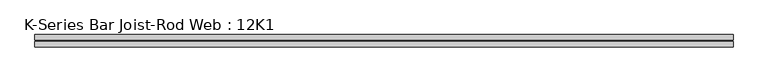
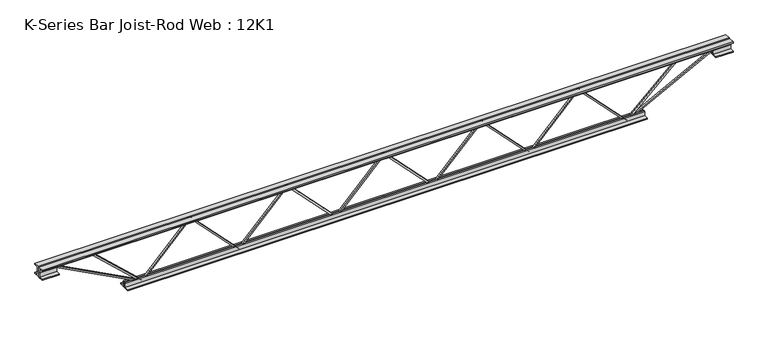
"""IFC4 building model written with IfcOpenShell, lengths in millimetres: beam geometry, K-Series Bar Joist-Rod Web : 12K1."""

from ifc_helpers import new_model, si_unit, frame, origin, place, context, project, spatial, polyline, outline, extrude, source, transform, mapped, element, save


def k_series_bar_joist_rod_web_12k1_6bf771c6(model_context):
    return source(origin(), model_context, "Body", "SweptSolid", [
        extrude(outline(polyline([(-141.2875, 287.02), (-150.8125, 287.02), (-150.8125, 292.22359), (141.2875, 572.89359), (141.2875, 575.18641), (-150.8125, 855.85641), (-150.8125, 861.06), (-141.2875, 861.06), (-141.2875, 859.91359), (150.8125, 579.24359), (150.8125, 568.83641), (-141.2875, 288.16641), (-141.2875, 287.02)])), frame((0.0, -4.7625, 0.0), z_axis=(0.0, 1.0, 0.0), x_axis=(0.0, 0.0, 1.0)), (0.0, 0.0, 1.0), 9.525),
        extrude(outline(polyline([(-141.2875, -287.02), (-150.8125, -287.02), (-150.8125, -281.81641), (141.2875, -1.14641), (141.2875, 1.14641), (-150.8125, 281.81641), (-150.8125, 287.02), (-141.2875, 287.02), (-141.2875, 285.87359), (150.8125, 5.20359), (150.8125, -5.20359), (-141.2875, -285.87359), (-141.2875, -287.02)])), frame((0.0, -4.7625, 0.0), z_axis=(0.0, 1.0, 0.0), x_axis=(0.0, 0.0, 1.0)), (0.0, 0.0, 1.0), 9.525),
        extrude(outline(polyline([(-141.2875, -861.06), (-150.8125, -861.06), (-150.8125, -855.85641), (141.2875, -575.18641), (141.2875, -572.89359), (-150.8125, -292.22359), (-150.8125, -287.02), (-141.2875, -287.02), (-141.2875, -288.16641), (150.8125, -568.83641), (150.8125, -579.24359), (-141.2875, -859.91359), (-141.2875, -861.06)])), frame((0.0, -4.7625, 0.0), z_axis=(0.0, 1.0, 0.0), x_axis=(0.0, 0.0, 1.0)), (0.0, 0.0, 1.0), 9.525),
        extrude(outline(polyline([(-141.2875, 861.06), (-150.8125, 861.06), (-150.8125, 866.26359), (141.2875, 1146.93359), (141.2875, 1149.22641), (-150.8125, 1429.89641), (-150.8125, 1435.1), (-141.2875, 1435.1), (-141.2875, 1433.95359), (150.8125, 1153.28359), (150.8125, 1142.87641), (-141.2875, 862.20641), (-141.2875, 861.06)])), frame((0.0, -4.7625, 0.0), z_axis=(0.0, 1.0, 0.0), x_axis=(0.0, 0.0, 1.0)), (0.0, 0.0, 1.0), 9.525),
        extrude(outline(polyline([(-141.2875, -1435.1), (-150.8125, -1435.1), (-150.8125, -1429.89641), (141.2875, -1149.22641), (141.2875, -1146.93359), (-150.8125, -866.26359), (-150.8125, -861.06), (-141.2875, -861.06), (-141.2875, -862.20641), (150.8125, -1142.87641), (150.8125, -1153.28359), (-141.2875, -1433.95359), (-141.2875, -1435.1)])), frame((0.0, -4.7625, 0.0), z_axis=(0.0, 1.0, 0.0), x_axis=(0.0, 0.0, 1.0)), (0.0, 0.0, 1.0), 9.525),
        extrude(outline(polyline([(4.7625, 152.4), (36.5125, 152.4), (36.5125, 146.05), (11.1125, 146.05), (11.1125, 120.65), (4.7625, 120.65), (4.7625, 152.4)])), frame((-2044.7, 0.0, 0.0), z_axis=(1.0, 0.0, 0.0), x_axis=(0.0, 1.0, 0.0)), (0.0, 0.0, 1.0), 4089.4),
        extrude(outline(polyline([(-4.7625, 152.4), (-4.7625, 120.65), (-11.1125, 120.65), (-11.1125, 146.05), (-36.5125, 146.05), (-36.5125, 152.4), (-4.7625, 152.4)])), frame((-2044.7, 0.0, 0.0), z_axis=(1.0, 0.0, 0.0), x_axis=(0.0, 1.0, 0.0)), (0.0, 0.0, 1.0), 4089.4),
        extrude(outline(polyline([(-4.7625, 88.9), (-36.5125, 88.9), (-36.5125, 95.25), (-11.1125, 95.25), (-11.1125, 120.65), (-4.7625, 120.65), (-4.7625, 88.9)])), frame((-2044.7, 0.0, 0.0), z_axis=(1.0, 0.0, 0.0), x_axis=(0.0, 1.0, 0.0)), (0.0, 0.0, 1.0), 101.6),
        extrude(outline(polyline([(36.5125, 88.9), (4.7625, 88.9), (4.7625, 120.65), (11.1125, 120.65), (11.1125, 95.25), (36.5125, 95.25), (36.5125, 88.9)])), frame((-2044.7, 0.0, 0.0), z_axis=(1.0, 0.0, 0.0), x_axis=(0.0, 1.0, 0.0)), (0.0, 0.0, 1.0), 101.6),
        extrude(outline(polyline([(4.7625, 88.9), (4.7625, 120.65), (11.1125, 120.65), (11.1125, 95.25), (36.5125, 95.25), (36.5125, 88.9), (4.7625, 88.9)])), frame((1943.1, 0.0, 0.0), z_axis=(1.0, 0.0, 0.0), x_axis=(0.0, 1.0, 0.0)), (0.0, 0.0, 1.0), 101.6),
        extrude(outline(polyline([(-4.7625, 88.9), (-36.5125, 88.9), (-36.5125, 95.25), (-11.1125, 95.25), (-11.1125, 120.65), (-4.7625, 120.65), (-4.7625, 88.9)])), frame((1943.1, 0.0, 0.0), z_axis=(1.0, 0.0, 0.0), x_axis=(0.0, 1.0, 0.0)), (0.0, 0.0, 1.0), 101.6),
        extrude(outline(polyline([(4.7625, -152.4), (4.7625, -120.65), (11.1125, -120.65), (11.1125, -146.05), (36.5125, -146.05), (36.5125, -152.4), (4.7625, -152.4)])), frame((-1536.7, 0.0, 0.0), z_axis=(1.0, 0.0, 0.0), x_axis=(0.0, 1.0, 0.0)), (0.0, 0.0, 1.0), 3073.4),
        extrude(outline(polyline([(-4.7625, -152.4), (-36.5125, -152.4), (-36.5125, -146.05), (-11.1125, -146.05), (-11.1125, -120.65), (-4.7625, -120.65), (-4.7625, -152.4)])), frame((-1536.7, 0.0, 0.0), z_axis=(1.0, 0.0, 0.0), x_axis=(0.0, 1.0, 0.0)), (0.0, 0.0, 1.0), 3073.4),
        extrude(outline(polyline([(0.0, -9.525), (0.0, 0.0), (573.7533355, 0.0), (573.7533355, -9.525), (0.0, -9.525)])), frame((-1945.3137714, 4.7625, 116.4332925), z_axis=(0.46483389898951466, 0.0, 0.8853979028381566), x_axis=(0.8853979028381566, 0.0, -0.46483389898951466)), (0.0, 0.0, 1.0), 9.525),
        extrude(outline(polyline([(0.0, -9.525), (0.0, 0.0), (391.8027187, 0.0), (391.8027187, -9.525), (0.0, -9.525)])), frame((-1725.3618324, 4.7625, 117.1611708), z_axis=(0.680699717623211, 0.0, 0.7325625532524037), x_axis=(0.7325625532524037, 0.0, -0.680699717623211)), (0.0, 0.0, 1.0), 9.525),
        extrude(outline(polyline([(0.0, -9.525), (0.0, 0.0), (573.7533355, 0.0), (573.7533355, -9.525), (0.0, -9.525)])), frame((1945.3137714, -4.7625, 116.4332925), z_axis=(-0.4648338989894953, 0.0, 0.8853979028381668), x_axis=(-0.8853979028381668, 0.0, -0.4648338989894953)), (0.0, 0.0, 1.0), 9.525),
        extrude(outline(polyline([(0.0, -9.525), (0.0, 0.0), (391.8027187, 0.0), (391.8027187, -9.525), (0.0, -9.525)])), frame((1725.3618324, -4.7625, 117.1611708), z_axis=(-0.6806997176232048, 0.0, 0.7325625532524095), x_axis=(-0.7325625532524095, 0.0, -0.6806997176232048)), (0.0, 0.0, 1.0), 9.525),
    ])


if __name__ == "__main__":
    model = new_model("IFC4")
    model_context = context("Model", 3, world=origin())
    ifc_project = project(units=[si_unit("LENGTHUNIT", "METRE", prefix="MILLI")], contexts=[model_context])
    site = spatial("IfcSite", under=ifc_project)
    building = spatial("IfcBuilding", under=site)
    placement = place(None, origin())
    k_series_bar_joist_rod_web_12k1_shape = k_series_bar_joist_rod_web_12k1_6bf771c6(model_context)
    element("IfcBeam", 1, ObjectType="K-Series Bar Joist-Rod Web : 12K1", at=placement, inside=building, context=model_context, shape_type="MappedRepresentation", body=[
        mapped(k_series_bar_joist_rod_web_12k1_shape, transform((0.0, 0.0, 0.0), x_axis=(1.0, 0.0, 0.0), y_axis=(0.0, 1.0, 0.0), z_axis=(0.0, 0.0, 1.0))),
    ])
    save(model, "model.ifc")

# Revit data of these elements
# Type "K-Series Bar Joist-Rod Web : 12K1"
#   Assembly Code = "B1010350"
#   Wt = 5
#   Web Thickness = 0' - 0 3/8"
#   Start Offset [instance default] = 0' - 0"
#   Start Extension [instance default] = 0' - 0"
#   Seat Length = 0' - 4"
#   Seat Depth = 0' - 2 1/2"
#   PanelArrayLength [instance default] = 20' - 0"
#   Panel [instance default] = 2' - 0"
#   End Offset [instance default] = 0' - 0"
#   End Extension [instance default] = 0' - 0"
#   End Panel = 2' - 0"
#   Cord Leg = 0' - 1 1/4"
#   Chord Thickness = 0' - 0 1/4"
#   Length [instance default] = 24' - 0"
#   Depth = 1' - 0"
#   PanelArrayNum [instance default] = 10
#   Structural Material = none
# Element 1 (IfcBeam, "K-Series Bar Joist-Rod Web : 12K1")
#   PanelArrayLength = 9' - 5"
#   Panel = 1' - 10.6"
#   PanelArrayNum = 5
